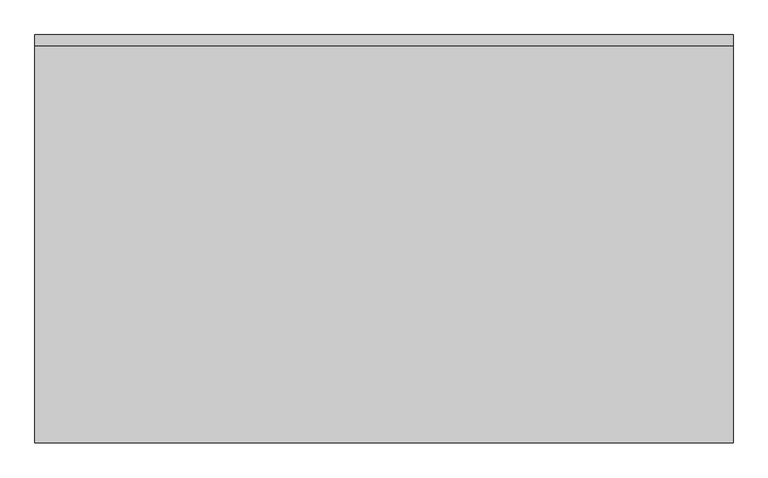
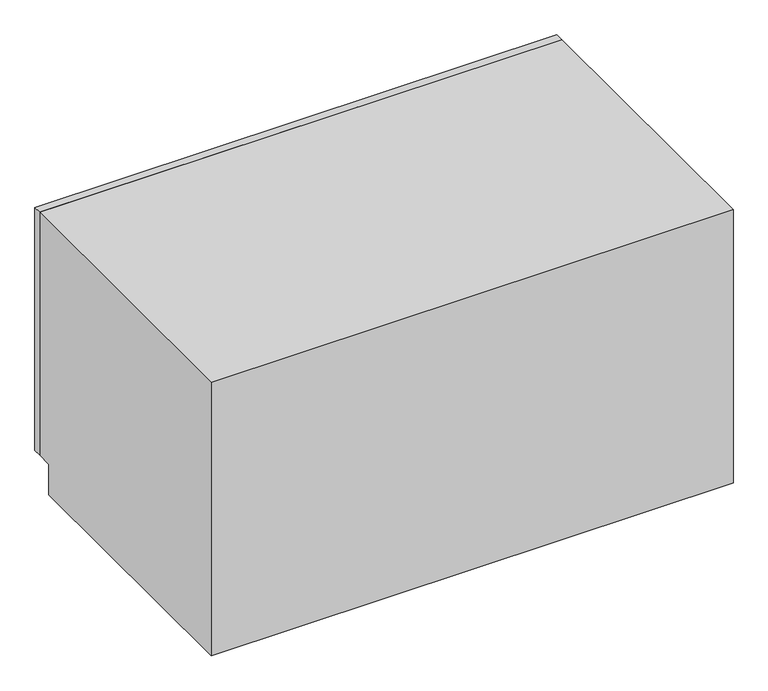
"""IFC4 building model written with IfcOpenShell, lengths in millimetres: furniture geometry, OD_CW_Base Cabinet : OD_CW_Base Cabinet."""

from ifc_helpers import new_model, si_unit, frame, origin, place, context, project, spatial, polyline, outline, extrude, source, transform, mapped, element, save


def furniture_39ad3696(model_context):
    return source(origin(), model_context, "Body", "SweptSolid", [
        extrude(outline(polyline([(18.7377049, 330.2), (18.7377049, 355.6), (1669.7377049, 355.6), (1669.7377049, 330.2), (18.7377049, 330.2)])), frame((0.0, 0.0, 101.6), z_axis=(0.0, 0.0, 1.0), x_axis=(1.0, 0.0, 0.0)), (0.0, 0.0, 1.0), 812.8),
        extrude(outline(polyline([(330.2, 914.4), (330.2, 101.6), (279.4, 101.6), (279.4, 0.0), (-609.6, 0.0), (-609.6, 914.4), (330.2, 914.4)])), frame((18.7377049, 0.0, 0.0), z_axis=(1.0, 0.0, 0.0), x_axis=(0.0, 1.0, 0.0)), (0.0, 0.0, 1.0), 1651.0),
    ])


if __name__ == "__main__":
    model = new_model("IFC4")
    model_context = context("Model", 3, world=origin())
    ifc_project = project(units=[si_unit("LENGTHUNIT", "METRE", prefix="MILLI")], contexts=[model_context])
    site = spatial("IfcSite", under=ifc_project)
    building = spatial("IfcBuilding", under=site)
    placement = place(None, origin())
    furniture_shape = furniture_39ad3696(model_context)
    element("IfcFurniture", 1, ObjectType="OD_CW_Base Cabinet : OD_CW_Base Cabinet", at=placement, inside=building, context=model_context, shape_type="MappedRepresentation", body=[
        mapped(furniture_shape, transform((0.0, 0.0, 0.0), x_axis=(1.0, 0.0, 0.0), y_axis=(0.0, 1.0, 0.0), z_axis=(0.0, 0.0, 1.0))),
    ])
    save(model, "model.ifc")

# Revit data of these elements
# Type "OD_CW_Base Cabinet : OD_CW_Base Cabinet"
#   OD_CW_Width [instance default] = 2' - 10"
#   OD_CW_Length [instance default] = 8' - 0"
#   OD_CW_Height [instance default] = 2' - 3"
#   Depth = 2' - 0"
#   Height = 3' - 0"
#   Width = 4' - 0"
#   OD_CW_Material_Front Panel [instance default] = none
#   OD_CW_Material_Body [instance default] = none
# Element 1 (IfcFurniture, "OD_CW_Base Cabinet : OD_CW_Base Cabinet")
#   OD_CW_Width = 3' - 2"
#   OD_CW_Length = 5' - 5"
#   OD_CW_Height = 3' - 0"
#   OD_CW_Material_Body = DISH MACHINE
#   Materials on its faces: "DISH MACHINE", "CASEWORK"
# Materials
#   "DISH MACHINE": class "Generic", colour RGB 187 187 187, transparency 0, Cost = 0
#   "CASEWORK": class "Generic", colour RGB 181 181 181, transparency 0, Cost = 0
